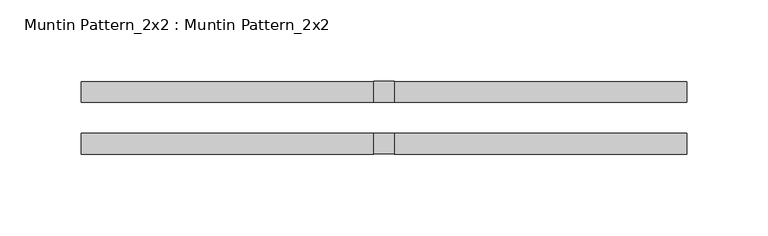
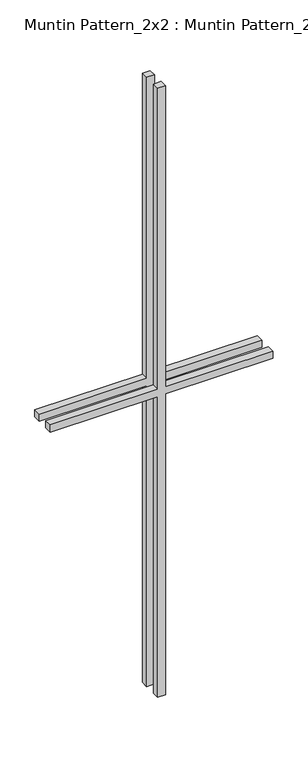
"""IFC4 building model written with IfcOpenShell, lengths in millimetres: proxy geometry, Muntin Pattern_2x2 : Muntin Pattern_2x2."""

from ifc_helpers import new_model, si_unit, frame, origin, place, context, project, spatial, polyline, outline, extrude, source, transform, mapped, element, save


def muntin_pattern_2x2_muntin_pattern_2x2_764e8cbb(model_context):
    return source(origin(), model_context, "Body", "SweptSolid", [
        extrude(outline(polyline([(542.925, -6.35), (542.925, -185.7375), (530.225, -185.7375), (530.225, -6.35), (0.0, -6.35), (0.0, 6.35), (530.225, 6.35), (530.225, 185.7375), (542.925, 185.7375), (542.925, 6.35), (1073.15, 6.35), (1073.15, -6.35), (542.925, -6.35)])), frame((0.0, -22.225, 0.0), z_axis=(0.0, 1.0, 0.0), x_axis=(0.0, 0.0, 1.0)), (0.0, 0.0, 1.0), 12.7),
        extrude(outline(polyline([(542.925, -6.35), (542.925, -185.7375), (530.225, -185.7375), (530.225, -6.35), (0.0, -6.35), (0.0, 6.35), (530.225, 6.35), (530.225, 185.7375), (542.925, 185.7375), (542.925, 6.35), (1073.15, 6.35), (1073.15, -6.35), (542.925, -6.35)])), frame((0.0, 9.525, 0.0), z_axis=(0.0, 1.0, 0.0), x_axis=(0.0, 0.0, 1.0)), (0.0, 0.0, 1.0), 12.7),
    ])


if __name__ == "__main__":
    model = new_model("IFC4")
    model_context = context("Model", 3, world=origin())
    ifc_project = project(units=[si_unit("LENGTHUNIT", "METRE", prefix="MILLI")], contexts=[model_context])
    site = spatial("IfcSite", under=ifc_project)
    building = spatial("IfcBuilding", under=site)
    placement = place(None, origin())
    muntin_pattern_2x2_muntin_pattern_2x2_shape = muntin_pattern_2x2_muntin_pattern_2x2_764e8cbb(model_context)
    element("IfcBuildingElementProxy", 1, Name="Muntin Pattern_2x2 : Muntin Pattern_2x2", ObjectType="Muntin Pattern_2x2 : Muntin Pattern_2x2", at=placement, inside=building, context=model_context, shape_type="MappedRepresentation", body=[
        mapped(muntin_pattern_2x2_muntin_pattern_2x2_shape, transform((0.0, 0.0, 0.0), x_axis=(1.0, 0.0, 0.0), y_axis=(0.0, 1.0, 0.0), z_axis=(0.0, 0.0, 1.0))),
    ])
    save(model, "model.ifc")

# Revit data of these elements
# Type "Muntin Pattern_2x2 : Muntin Pattern_2x2"
#   Width [instance default] = 4' - 0"
#   Thickness = 0' - 0 1/2"
#   Height [instance default] = 4' - 0"
#   Distance = 0' - 0 3/4"
#   Interior Material [instance default] = none
#   Exterior Material [instance default] = none
#   Default Elevation = 0
# Element 1 (IfcBuildingElementProxy, "Muntin Pattern_2x2 : Muntin Pattern_2x2")
#   Width = 1' - 2 5/8"
#   Height = 3' - 6 1/4"
#   Interior Material = Wood - Stained
#   Exterior Material = Clad - White
#   Materials on its faces: "Clad - White", "Wood - Stained"
# Materials
#   "Clad - White": class "Wood", colour RGB 242 242 238, transparency 0, Cost = 0
#   "Wood - Stained": class "Wood", colour RGB 224 178 126, transparency 0, Cost = 0
